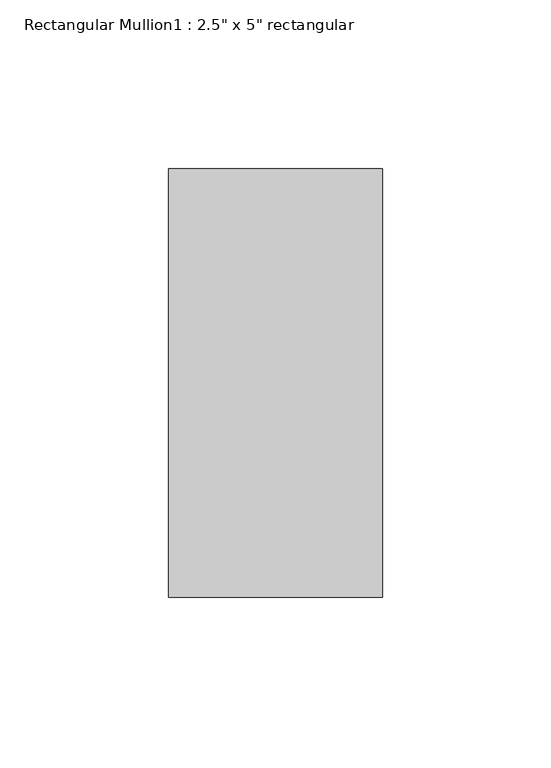
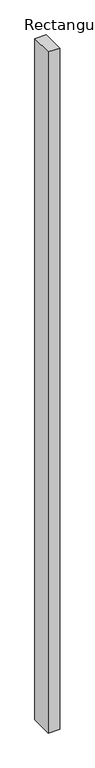
"""IFC4 building model written with IfcOpenShell, lengths in millimetres: member geometry."""

from ifc_helpers import new_model, si_unit, frame, origin, place, context, project, spatial, polyline, outline, extrude, source, transform, mapped, element, save


def member_01a33192(model_context):
    return source(origin(), model_context, "Body", "SweptSolid", [
        extrude(outline(polyline([(31.75, 63.5), (31.75, -63.5), (-31.75, -63.5), (-31.75, 63.5), (31.75, 63.5)])), frame((0.0, 0.0, -3971.7835741), z_axis=(0.0, 0.0, 1.0), x_axis=(1.0, 0.0, 0.0)), (0.0, 0.0, 1.0), 3971.7835741),
    ])


if __name__ == "__main__":
    model = new_model("IFC4")
    model_context = context("Model", 3, world=origin())
    ifc_project = project(units=[si_unit("LENGTHUNIT", "METRE", prefix="MILLI")], contexts=[model_context])
    site = spatial("IfcSite", under=ifc_project)
    building = spatial("IfcBuilding", under=site)
    placement = place(None, origin())
    member_shape = member_01a33192(model_context)
    element("IfcMember", 1, ObjectType="Rectangular Mullion1 : 2.5\" x 5\" rectangular", at=placement, inside=building, context=model_context, shape_type="MappedRepresentation", body=[
        mapped(member_shape, transform((0.0, 0.0, 0.0), x_axis=(1.0, 0.0, 0.0), y_axis=(0.0, 1.0, 0.0), z_axis=(0.0, 0.0, 1.0))),
    ])
    save(model, "model.ifc")

# Revit data of these elements
# Type "Rectangular Mullion1 : 2.5\" x 5\" rectangular"
#   built-in parameter 1007304 = 0.416667 (stored number, unit not read)
#   built-in parameter 1007301 = 0.104167 (stored number, unit not read)
#   built-in parameter 1007300 = 0.104167 (stored number, unit not read)
# Element 1 (IfcMember, "Rectangular Mullion1 : 2.5\" x 5\" rectangular")
#   Materials on its faces: "support-frame"
# Materials
#   "support-frame": class "Unassigned", colour RGB 233 233 233, transparency 0, Cost = 0
